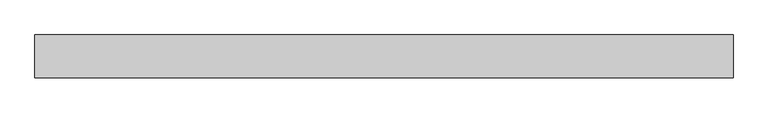
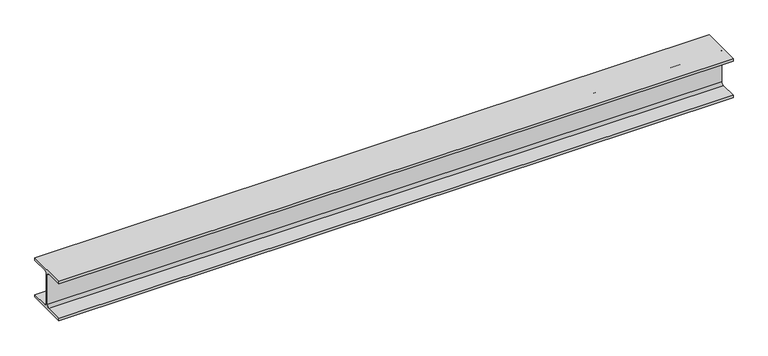
"""IFC4 building model written with IfcOpenShell, lengths in millimetres: beam geometry, 0912_Steel Framing_H-KSD3502 : H_SB_ASB_H-200x200x8x12."""

import ifcopenshell
import ifcopenshell.guid

model = None  # the IFC model being written
_history = None  # IfcOwnerHistory: only IFC2X3 demands one
_inside = {}  # id of a spatial element -> (the spatial element, [elements in it])
_under = {}  # id of a project, library or spatial element -> (it, [spatial elements below it])
_declared = {}  # id of a project -> (the project, [libraries it declares])
_typed = {}  # id of a type object -> (the type object, [elements of that type])
_made_of = {}  # id of a material, layer set ... -> (it, [elements and type objects made of it])


def new_model(schema):
    """Start an empty IFC model of exactly this schema.

    Asked for "IFC4X3", IfcOpenShell would pick the latest addendum, in which some entities
    have other attributes; the version numbers below select the first issue.
    IFC2X3 requires an IfcOwnerHistory on every rooted entity: one is made here for all.
    """
    global model, _history
    if schema == "IFC4X3":
        model = ifcopenshell.file(schema_version=(4, 3, 0, 0))
    else:
        model = ifcopenshell.file(schema=schema)
    _inside.clear()
    _under.clear()
    _declared.clear()
    _typed.clear()
    _made_of.clear()
    _history = None
    if model.schema == "IFC2X3":
        org = make("IfcOrganization", Name="unknown")
        user = make(
            "IfcPersonAndOrganization",
            ThePerson=make("IfcPerson", FamilyName="unknown"),
            TheOrganization=org,
        )
        app = make(
            "IfcApplication",
            ApplicationDeveloper=org,
            Version="unknown",
            ApplicationFullName="unknown",
            ApplicationIdentifier="unknown",
        )
        _history = make(
            "IfcOwnerHistory",
            OwningUser=user,
            OwningApplication=app,
            ChangeAction="ADDED",
            CreationDate=0,
        )
    return model


def make(cls, **values):
    """One entity of the class cls with the attributes given. An attribute that is None is left unset."""
    return model.create_entity(
        cls, **{name: value for name, value in values.items() if value is not None}
    )


def rooted(cls, **values):
    """An entity with a GlobalId (a new one), such as an element, a storey or a relation."""
    return make(cls, GlobalId=ifcopenshell.guid.new(), OwnerHistory=_history, **values)


def si_unit(unit_type, name, prefix=None):
    """IfcSIUnit, for example si_unit("LENGTHUNIT", "METRE", prefix="MILLI")."""
    return make("IfcSIUnit", UnitType=unit_type, Prefix=prefix, Name=name)


def assignment(units):
    """IfcUnitAssignment: the units of a project."""
    return None if units is None else make("IfcUnitAssignment", Units=units)


def point(xyz):
    """IfcCartesianPoint."""
    return None if xyz is None else make("IfcCartesianPoint", Coordinates=xyz)


def direction(xyz):
    """IfcDirection."""
    return None if xyz is None else make("IfcDirection", DirectionRatios=xyz)


def frame(location, z_axis=None, x_axis=None):
    """IfcAxis2Placement3D, a coordinate frame: its origin and axes. An axis left out is left unset."""
    return make(
        "IfcAxis2Placement3D",
        Location=point(location),
        Axis=direction(z_axis),
        RefDirection=direction(x_axis),
    )


def frame_2d(location, x_axis=None):
    """IfcAxis2Placement2D, a coordinate frame in the plane: its origin and x axis."""
    return make(
        "IfcAxis2Placement2D", Location=point(location), RefDirection=direction(x_axis)
    )


def origin():
    """The frame at (0, 0, 0) with its axes left unset."""
    return frame((0.0, 0.0, 0.0))


def place(relative_to, where):
    """IfcLocalPlacement: puts the frame where relative to a parent placement (None: the world)."""
    return make(
        "IfcLocalPlacement", PlacementRelTo=relative_to, RelativePlacement=where
    )


def context(
    kind, dimensions, precision=None, world=None, true_north=None, identifier=None
):
    """IfcGeometricRepresentationContext, for example the 3D "Model" context."""
    return make(
        "IfcGeometricRepresentationContext",
        ContextIdentifier=identifier,
        ContextType=kind,
        CoordinateSpaceDimension=dimensions,
        Precision=precision,
        WorldCoordinateSystem=world,
        TrueNorth=true_north,
    )


def project(units=None, contexts=None):
    """IfcProject with its units and contexts."""
    return rooted(
        "IfcProject",
        Name="project",
        RepresentationContexts=contexts,
        UnitsInContext=assignment(units),
    )


def spatial(cls, under=None, at=None, **own):
    """A site, building, storey or space (cls), placed at a placement, below another one or the project."""
    s = rooted(cls, ObjectPlacement=at, **own)
    if under is not None:
        _under.setdefault(under.id(), (under, []))[1].append(s)
    return s


def polyline(points):
    """IfcPolyline through the points."""
    return make("IfcPolyline", Points=[point(p) for p in points])


def circle_curve(where, radius):
    """IfcCircle in the frame where."""
    return make("IfcCircle", Position=where, Radius=radius)


def trimmed(basis, trim1, trim2, sense, master):
    """IfcTrimmedCurve: the piece of a basis curve between two trims."""
    return make(
        "IfcTrimmedCurve",
        BasisCurve=basis,
        Trim1=trim1,
        Trim2=trim2,
        SenseAgreement=sense,
        MasterRepresentation=master,
    )


def segment(curve, same_sense, transition):
    """IfcCompositeCurveSegment."""
    return make(
        "IfcCompositeCurveSegment",
        Transition=transition,
        SameSense=same_sense,
        ParentCurve=curve,
    )


def composite_curve(segments, self_intersect=None):
    """IfcCompositeCurve: segments joined end to end."""
    return make("IfcCompositeCurve", Segments=segments, SelfIntersect=self_intersect)


def outline(outer, holes=None, kind="AREA"):
    """IfcArbitraryClosedProfileDef: a profile drawn as a closed curve; with holes, ...WithVoids."""
    if holes is None:
        return make("IfcArbitraryClosedProfileDef", ProfileType=kind, OuterCurve=outer)
    return make(
        "IfcArbitraryProfileDefWithVoids",
        ProfileType=kind,
        OuterCurve=outer,
        InnerCurves=holes,
    )


def extrude(swept, where, along, depth):
    """IfcExtrudedAreaSolid: the profile swept, set in the frame where, extruded along a direction by depth."""
    return make(
        "IfcExtrudedAreaSolid",
        SweptArea=swept,
        Position=where,
        ExtrudedDirection=direction(along),
        Depth=depth,
    )


def shape(context_of_items, identifier, shape_type, items):
    """IfcShapeRepresentation: the items that make up one representation, for example the "Body"."""
    return make(
        "IfcShapeRepresentation",
        ContextOfItems=context_of_items,
        RepresentationIdentifier=identifier,
        RepresentationType=shape_type,
        Items=items,
    )


def source(mapping_origin, context_of_items, identifier, shape_type, items):
    """IfcRepresentationMap: a shape defined once, which mapped items show again and again."""
    return make(
        "IfcRepresentationMap",
        MappingOrigin=mapping_origin,
        MappedRepresentation=shape(context_of_items, identifier, shape_type, items),
    )


def transform(
    local_origin,
    x_axis=None,
    y_axis=None,
    z_axis=None,
    scale=None,
    scale2=None,
    scale3=None,
    uniform=True,
):
    """IfcCartesianTransformationOperator3D, or its non-uniform kind. x_axis, y_axis, z_axis: its Axis1, 2, 3."""
    if uniform:
        return make(
            "IfcCartesianTransformationOperator3D",
            Axis1=direction(x_axis),
            Axis2=direction(y_axis),
            LocalOrigin=point(local_origin),
            Scale=scale,
            Axis3=direction(z_axis),
        )
    return make(
        "IfcCartesianTransformationOperator3DnonUniform",
        Axis1=direction(x_axis),
        Axis2=direction(y_axis),
        LocalOrigin=point(local_origin),
        Scale=scale,
        Axis3=direction(z_axis),
        Scale2=scale2,
        Scale3=scale3,
    )


def mapped(mapping_source, mapping_target):
    """IfcMappedItem: shows the shape of a source again, moved by a transform."""
    return make(
        "IfcMappedItem", MappingSource=mapping_source, MappingTarget=mapping_target
    )


def made_of(thing, what):
    """Note that an element or type object is made of a material, layer set ...; save() writes the relation."""
    if what is not None:
        _made_of.setdefault(what.id(), (what, []))[1].append(thing)
    return thing


def element(
    cls,
    number,
    at=None,
    inside=None,
    cuts=None,
    type_object=None,
    material=None,
    context=None,
    identifier="Body",
    shape_type=None,
    held_by="IfcProductDefinitionShape",
    body=None,
    shapes=None,
    **own,
):
    """One element of the class cls, such as IfcWall. Its Tag is "e" and its number.

    at: its placement. inside: the storey or other place that contains it. cuts: it is an
    opening in that element (IfcRelVoidsElement). A single representation is given by context,
    identifier, shape_type and body (its items); several are given by shapes. held_by: the class
    of the entity that holds the representations. save() writes the other relations.
    """
    e = rooted(cls, Tag="e%d" % number, ObjectPlacement=at, **own)
    if body is not None:
        shapes = [shape(context, identifier, shape_type, body)]
    if shapes is not None:
        e.Representation = make(held_by, Representations=shapes)
    if inside is not None:
        _inside.setdefault(inside.id(), (inside, []))[1].append(e)
    if cuts is not None:
        rooted(
            "IfcRelVoidsElement", RelatingBuildingElement=cuts, RelatedOpeningElement=e
        )
    if type_object is not None:
        _typed.setdefault(type_object.id(), (type_object, []))[1].append(e)
    return made_of(e, material)


def aggregate(whole, parts):
    """IfcRelAggregates: a whole, such as a stair, and the parts it consists of."""
    return rooted("IfcRelAggregates", RelatingObject=whole, RelatedObjects=parts)


def save(model, path):
    """Write the relations noted so far, then the file.

    IfcRelAggregates (storeys below a building ...), IfcRelContainedInSpatialStructure (elements
    in a storey), IfcRelDefinesByType, IfcRelAssociatesMaterial and IfcRelDeclares: one each for
    every whole, place, type object, material and project.
    """
    for whole, parts in _under.values():
        aggregate(whole, parts)
    for where, things in _inside.values():
        rooted(
            "IfcRelContainedInSpatialStructure",
            RelatedElements=things,
            RelatingStructure=where,
        )
    for kind, things in _typed.values():
        rooted("IfcRelDefinesByType", RelatedObjects=things, RelatingType=kind)
    for what, things in _made_of.values():
        rooted("IfcRelAssociatesMaterial", RelatedObjects=things, RelatingMaterial=what)
    for by, libraries in _declared.values():
        rooted("IfcRelDeclares", RelatingContext=by, RelatedDefinitions=libraries)
    model.write(path)


def beam_3af3bc90(model_context):
    return source(origin(), model_context, "Body", "SweptSolid", [
        extrude(outline(composite_curve([segment(polyline([(100.0, -88.0), (100.0, -100.0), (-100.0, -100.0), (-100.0, -88.0), (-17.0, -88.0)]), True, "CONTINUOUS"), segment(trimmed(circle_curve(frame_2d((-17.0, -75.0)), 13.0), [point((-17.0, -88.0))], [point((-4.0, -75.0))], True, "CARTESIAN"), True, "CONTINUOUS"), segment(polyline([(-4.0, -75.0), (-4.0, 75.0)]), True, "CONTINUOUS"), segment(trimmed(circle_curve(frame_2d((-17.0, 75.0)), 13.0), [point((-4.0, 75.0))], [point((-17.0, 88.0))], True, "CARTESIAN"), True, "CONTINUOUS"), segment(polyline([(-17.0, 88.0), (-100.0, 88.0), (-100.0, 100.0), (100.0, 100.0), (100.0, 88.0), (17.0, 88.0)]), True, "CONTINUOUS"), segment(trimmed(circle_curve(frame_2d((17.0, 75.0)), 13.0), [point((17.0, 88.0))], [point((4.0, 75.0))], True, "CARTESIAN"), True, "CONTINUOUS"), segment(polyline([(4.0, 75.0), (4.0, -75.0)]), True, "CONTINUOUS"), segment(trimmed(circle_curve(frame_2d((17.0, -75.0)), 13.0), [point((4.0, -75.0))], [point((17.0, -88.0))], True, "CARTESIAN"), True, "CONTINUOUS"), segment(polyline([(17.0, -88.0), (100.0, -88.0)]), True, "CONTINUOUS")], self_intersect=False)), frame((-1681.1050298, 0.0, 0.0), z_axis=(1.0, 0.0, 0.0), x_axis=(0.0, 1.0, 0.0)), (0.0, 0.0, 1.0), 3257.9090537),
    ])


if __name__ == "__main__":
    model = new_model("IFC4")
    model_context = context("Model", 3, world=origin())
    ifc_project = project(units=[si_unit("LENGTHUNIT", "METRE", prefix="MILLI")], contexts=[model_context])
    site = spatial("IfcSite", under=ifc_project)
    building = spatial("IfcBuilding", under=site)
    placement = place(None, origin())
    beam_shape = beam_3af3bc90(model_context)
    element("IfcBeam", 1, ObjectType="0912_Steel Framing_H-KSD3502 : H_SB_ASB_H-200x200x8x12", at=placement, inside=building, context=model_context, shape_type="MappedRepresentation", body=[
        mapped(beam_shape, transform((0.0, 0.0, 0.0), x_axis=(1.0, 0.0, 0.0), y_axis=(0.0, 1.0, 0.0), z_axis=(0.0, 0.0, 1.0))),
    ])
    save(model, "model.ifc")

# Revit data of these elements
# Type "0912_Steel Framing_H-KSD3502 : H_SB_ASB_H-200x200x8x12"
#   H_WM Code_1 = "S01AA002-00001 | Main Steel Structure Fabrication Work | Shelter/Building | Medium Steel - Standard (90KG/M>Weight≥30KG/M) | Material: (   )"
#   H_WM Code_2 = "S03AA028-00001 | Main Steel Structure Erection Work | Shelter/Building | Medium Steel (90KG/M>Weight≥30KG/M) | Material: (   )"
#   H_WM Code_3 = "S01AA010-00001 | Main Steel Structure Fabrication Work | Shelter/Building | Steel Painting/Coating | for Non-Fireproofed Steel Surface, Surface Preparation, Primer, Second & Final Coat | Material: (   )"
#   H_Q'ty Cal Type Tag = "SB-Q2"
#   Width = 20.0 cm
#   Web Thickness = 0.8 cm
#   Web Fillet = 1.3 cm
#   Warping Constant = 141000.0 cm⁶
#   W = 0
#   Torsional Moment of Inertia = 26.2485 cm⁴
#   Section Area = 63.53 cm²
#   Plastic Modulus weak axis = 244.0 cm³
#   Plastic Modulus strong axis = 525.0 cm³
#   Perimeter = 1.16 m²/m
#   Nominal Weight = 49.90 kgf/m
#   Moment of Inertia weak axis = 1600.00 cm⁴
#   Moment of Inertia strong axis = 4720.00 cm⁴
#   Height = 20.0 cm
#   Flange Thickness = 1.2 cm
#   Elastic Modulus weak axis = 160.0 cm³
#   Elastic Modulus strong axis = 472.0 cm³
#   Centroid Vertical = 10.0 cm
#   Centroid Horizontal = 10.0 cm
#   Ix = 47200000
#   Length [instance default] = 1.5240 m
#   Zx = 525000
#   b = 0.2000 m
#   h = 0.2000 m
#   r = 0.0130 m
#   s = 0.0080 m
#   t = 0.0120 m
#   A = 0.006353 m²
#   Structural Material [instance default] = Steel, 45-345
#   Assembly Code = ""
# Element 1 (IfcBeam, "0912_Steel Framing_H-KSD3502 : H_SB_ASB_H-200x200x8x12")
#   Structural Material = none
# Materials
#   "Steel, 45-345": class "Metal", colour RGB 189 187 185, transparency 0, Description = "Steel 345 MPa", Cost = 0
